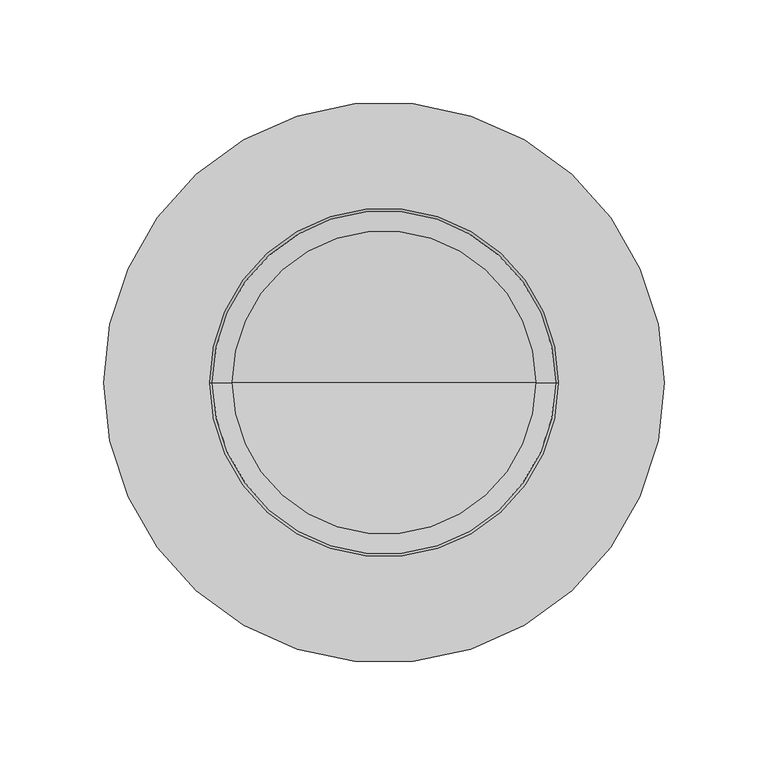
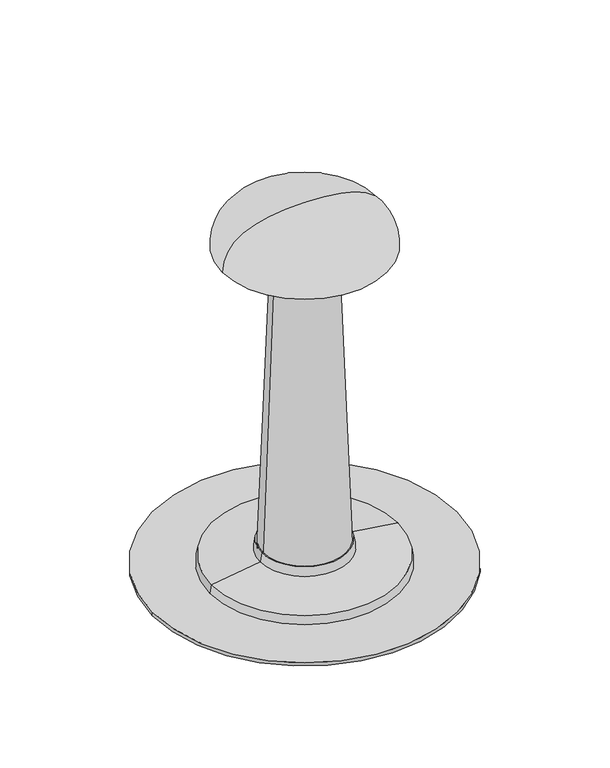
"""IFC4 building model written with IfcOpenShell, lengths in millimetres: proxy geometry, TN_Аэратор кровельный ТехноНИКОЛЬ ЭКО_Тип 1 : Аэратор кровельный ТехноНИКОЛЬ ЭКО 75х340мм."""

from ifc_helpers import new_model, si_unit, point, frame, origin, origin_with_axes, origin_2d, place, context, project, spatial, polyline, circle_curve, trimmed, segment, composite_curve, outline, extrude, source, transform, mapped, element, save
from ifc_brep_helpers import plane_surface, revolved_surface, spline_curve, advanced_brep


def specialty_equipment_94cada28(model_context):
    return source(origin(), model_context, "Body", "SolidModel", [
        advanced_brep(
        [(26.3779945, 0.0, 300.3783699), (-26.3779945, 0.0, 300.3783699), (0.0, 0.0, 300.3783699), (0.0, 0.0, 3.0), (-37.5, 0.0, 3.0), (37.5, 0.0, 3.0)],
        [
            (0, 1, circle_curve(frame((0.0, 0.0, 300.3783699), z_axis=(0.0, 0.0, 1.0), x_axis=(-1.0, 0.0, 0.0)), 26.3779945)),
            (1, 2),
            (2, 0),
            (1, 0, circle_curve(frame((0.0, 0.0, 300.3783699), z_axis=(0.0, 0.0, 1.0), x_axis=(-1.0, 0.0, 0.0)), 26.3779945)),
            (3, 4),
            (4, 5, circle_curve(frame((0.0, 0.0, 3.0), z_axis=(0.0, 0.0, -1.0), x_axis=(-1.0, 0.0, 0.0)), 37.5)),
            (5, 3),
            (5, 4, circle_curve(frame((0.0, 0.0, 3.0), z_axis=(0.0, 0.0, -1.0), x_axis=(-1.0, 0.0, 0.0)), 37.5)),
            (4, 1),
            (0, 5),
        ],
        [
            plane_surface(frame((0.0, 0.0, 300.3783699), z_axis=(0.0, 0.0, 1.0), x_axis=(-1.0, 0.0, 0.0))),
            plane_surface(frame((0.0, 0.0, 3.0), z_axis=(0.0, 0.0, -1.0), x_axis=(-1.0, 0.0, 0.0))),
            revolved_surface(polyline([(-26.3779945, 0.0, 300.3783699), (-37.5, 0.0, 3.0)]), (0.0, 0.0, 0.0), (0.0, 0.0, -1.0)),
        ],
        [
            (0, [[1, 2, 3]]),
            (0, [[4, -3, -2]]),
            (1, [[5, 6, 7]]),
            (1, [[-7, 8, -5]]),
            (2, [[-6, 9, -1, 10]]),
            (2, [[-8, -10, -4, -9]]),
        ],
    ),
        advanced_brep(
        [(0.0, 0.0, 300.3783699), (-73.0, 0.0, 300.3783699), (73.0, 0.0, 300.3783699), (0.0, 0.0, 340.3783699)],
        [
            (0, 1),
            (1, 2, circle_curve(frame((0.0, 0.0, 300.3783699), z_axis=(0.0, 0.0, -1.0), x_axis=(-1.0, 0.0, 0.0)), 73.0)),
            (2, 0),
            (2, 1, circle_curve(frame((0.0, 0.0, 300.3783699), z_axis=(0.0, 0.0, -1.0), x_axis=(-1.0, 0.0, 0.0)), 73.0)),
            (1, 3, spline_curve(3, [(-73.0, 0.0, 300.3783699), (-73.0, 0.0, 327.045036564), (-48.666666669, 0.0, 340.3783699), (0.0, 0.0, 340.3783699)], [4, 4], [0.0, 0.1853674540682417])),
            (3, 2, spline_curve(3, [(0.0, 0.0, 340.3783699), (48.666666669, 0.0, 340.3783699), (73.0, 0.0, 327.045036564), (73.0, 0.0, 300.3783699)], [4, 4], [0.0, 0.1853674540682417])),
        ],
        [
            plane_surface(frame((0.0, 0.0, 300.3783699), z_axis=(0.0, 0.0, -1.0), x_axis=(-1.0, 0.0, 0.0))),
            revolved_surface(spline_curve(3, [(0.0, 0.0, 340.3783699), (-48.666666669, 0.0, 340.3783699), (-73.0, 0.0, 327.045036564), (-73.0, 0.0, 300.3783699)], [4, 4], [0.0, 0.1853674540682417]), (0.0, 0.0, 340.3783699), (0.0, 0.0, -1.0)),
        ],
        [
            (0, [[1, 2, 3]]),
            (0, [[-3, 4, -1]]),
            (1, [[-2, 5, 6]]),
            (1, [[-4, -6, -5]]),
        ],
    ),
        advanced_brep(
        [(39.4106158, 0.0, 17.0), (-39.4106158, 0.0, 17.0), (-38.0, 0.0, 25.0), (38.0, 0.0, 25.0), (82.642123, 0.0, 10.7009033), (-82.642123, 0.0, 10.7009033), (84.0, 0.0, 3.0), (-84.0, 0.0, 3.0), (37.5, 0.0, 3.0), (-37.5, 0.0, 3.0), (-36.4162562, 0.0, 25.0), (36.4162562, 0.0, 25.0)],
        [
            (0, 1, circle_curve(frame((0.0, 0.0, 17.0), z_axis=(0.0, 0.0, 1.0), x_axis=(-1.0, 0.0, 0.0)), 39.4106158)),
            (1, 2),
            (2, 3, circle_curve(frame((0.0, 0.0, 25.0), z_axis=(0.0, 0.0, -1.0), x_axis=(-1.0, 0.0, 0.0)), 38.0)),
            (3, 0),
            (1, 0, circle_curve(frame((0.0, 0.0, 17.0), z_axis=(0.0, 0.0, 1.0), x_axis=(-1.0, 0.0, 0.0)), 39.4106158)),
            (3, 2, circle_curve(frame((0.0, 0.0, 25.0), z_axis=(0.0, 0.0, -1.0), x_axis=(-1.0, 0.0, 0.0)), 38.0)),
            (4, 5, circle_curve(frame((0.0, 0.0, 10.7009033), z_axis=(0.0, 0.0, 1.0), x_axis=(-1.0, 0.0, 0.0)), 82.642123)),
            (5, 1),
            (0, 4),
            (5, 4, circle_curve(frame((0.0, 0.0, 10.7009033), z_axis=(0.0, 0.0, 1.0), x_axis=(-1.0, 0.0, 0.0)), 82.642123)),
            (6, 7, circle_curve(frame((0.0, 0.0, 3.0), z_axis=(0.0, 0.0, 1.0), x_axis=(-1.0, 0.0, 0.0)), 84.0)),
            (7, 5),
            (4, 6),
            (7, 6, circle_curve(frame((0.0, 0.0, 3.0), z_axis=(0.0, 0.0, 1.0), x_axis=(-1.0, 0.0, 0.0)), 84.0)),
            (8, 9, circle_curve(frame((0.0, 0.0, 3.0), z_axis=(0.0, 0.0, 1.0), x_axis=(-1.0, 0.0, 0.0)), 37.5)),
            (9, 7),
            (6, 8),
            (9, 8, circle_curve(frame((0.0, 0.0, 3.0), z_axis=(0.0, 0.0, 1.0), x_axis=(-1.0, 0.0, 0.0)), 37.5)),
            (2, 10),
            (10, 11, circle_curve(frame((0.0, 0.0, 25.0), z_axis=(0.0, 0.0, -1.0), x_axis=(-1.0, 0.0, 0.0)), 36.4162562)),
            (11, 3),
            (11, 10, circle_curve(frame((0.0, 0.0, 25.0), z_axis=(0.0, 0.0, -1.0), x_axis=(-1.0, 0.0, 0.0)), 36.4162562)),
            (10, 9),
            (8, 11),
        ],
        [
            revolved_surface(polyline([(-38.0, 0.0, 25.0), (-39.4106158, 0.0, 17.0)]), (0.0, 0.0, 0.0), (0.0, 0.0, -1.0)),
            revolved_surface(polyline([(-39.4106158, 0.0, 17.0), (-82.642123, 0.0, 10.7009033)]), (0.0, 0.0, 0.0), (0.0, 0.0, -1.0)),
            revolved_surface(polyline([(-82.642123, 0.0, 10.7009033), (-84.0, 0.0, 3.0)]), (0.0, 0.0, 0.0), (0.0, 0.0, -1.0)),
            plane_surface(frame((0.0, 0.0, 3.0), z_axis=(0.0, 0.0, -1.0), x_axis=(-1.0, 0.0, 0.0))),
            plane_surface(frame((0.0, 0.0, 25.0), z_axis=(0.0, 0.0, 1.0), x_axis=(-1.0, 0.0, 0.0))),
            revolved_surface(polyline([(-37.5, 0.0, 3.0), (-36.4162562, 0.0, 25.0)]), (0.0, 0.0, 0.0), (0.0, 0.0, -1.0)),
        ],
        [
            (0, [[1, 2, 3, 4]]),
            (0, [[5, -4, 6, -2]]),
            (1, [[7, 8, -1, 9]]),
            (1, [[10, -9, -5, -8]]),
            (2, [[11, 12, -7, 13]]),
            (2, [[14, -13, -10, -12]]),
            (3, [[15, 16, -11, 17]]),
            (3, [[18, -17, -14, -16]]),
            (4, [[-3, 19, 20, 21]]),
            (4, [[-6, -21, 22, -19]]),
            (5, [[-20, 23, -15, 24]]),
            (5, [[-22, -24, -18, -23]]),
        ],
    ),
        extrude(outline(composite_curve([segment(trimmed(circle_curve(origin_2d(), 135.0), [point((-135.0, 0.0))], [point((135.0, 0.0))], False, "CARTESIAN"), True, "CONTINUOUS"), segment(trimmed(circle_curve(origin_2d(), 135.0), [point((135.0, 0.0))], [point((-135.0, 0.0))], False, "CARTESIAN"), True, "CONTINUOUS")], self_intersect=False)), origin_with_axes(), (0.0, 0.0, 1.0), 3.0),
    ])


if __name__ == "__main__":
    model = new_model("IFC4")
    model_context = context("Model", 3, world=origin())
    ifc_project = project(units=[si_unit("LENGTHUNIT", "METRE", prefix="MILLI")], contexts=[model_context])
    site = spatial("IfcSite", under=ifc_project)
    building = spatial("IfcBuilding", under=site)
    placement = place(None, origin())
    specialty_equipment_shape = specialty_equipment_94cada28(model_context)
    element("IfcBuildingElementProxy", 1, Name="TN_Аэратор кровельный ТехноНИКОЛЬ ЭКО_Тип 1 : Аэратор кровельный ТехноНИКОЛЬ ЭКО 75х340мм", ObjectType="TN_Аэратор кровельный ТехноНИКОЛЬ ЭКО_Тип 1 : Аэратор кровельный ТехноНИКОЛЬ ЭКО 75х340мм", at=placement, inside=building, context=model_context, shape_type="MappedRepresentation", body=[
        mapped(specialty_equipment_shape, transform((0.0, 0.0, 0.0), x_axis=(1.0, 0.0, 0.0), y_axis=(0.0, 1.0, 0.0), z_axis=(0.0, 0.0, 1.0))),
    ])
    save(model, "model.ifc")

# Revit data of these elements
# Type "TN_Аэратор кровельный ТехноНИКОЛЬ ЭКО_Тип 1 : Аэратор кровельный ТехноНИКОЛЬ ЭКО 75х340мм"
#   Description = "Аэратор кровельный ТехноНИКОЛЬ ЭКО 75х340 мм может быть использован только при\r\nремонтах кровли. Аэродинамическая форма и уменьшенное проходное сечение позволяют ему работать только после\r\nдостаточно сильного прогрева кровли. Устанавливается 1 на 100 м2 вне зависимости от способа монтажа кровли и\r\nпредотвращает только образование вздутий под кровлей. Его конструкция не подразумевает доутепления\r\nкерамзитовым гравием.\r\nКровельные аэраторы запрещено устанавливать в совмещенных кровлях над холодильниками и ледовыми аренами."
#   Manufacturer = "ТехноНИКОЛЬ"
#   URL = "https://shop.tn.ru/ajerator-krovel-nyj-tehnonikol-jeko-75h340-mm"
#   ADSK_Примечание = ""
#   ADSK_Обозначение = "ТехноНИКОЛЬ"
#   ADSK_Наименование = "Аэратор кровельный ТехноНИКОЛЬ ЭКО 75х340мм"
#   ADSK_Марка = ""
#   ADSK_Код изделия = "5489"
#   ADSK_Завод-изготовитель = "ТехноНИКОЛЬ"
#   ADSK_Единица измерения = "шт."
#   ADSK_Группирование = "Комплектующие и воронки"
#   ADSK_URL страницы изделия = "https://shop.tn.ru/ajerator-krovel-nyj-tehnonikol-jeko-75h340-mm#documents"
#   ADSK_URL документации изделия = "https://nav.tn.ru/upload/iblock/68a/Tekhlist-7.18_Aerator-krovelnyy-TekhnoNIKOL_rus.pdf"
#   ADSK_Масса = 0.3
#   ADSK_Количество = 1
#   Материал = TN_ПВХ_Черный
#   Default Elevation = 0
# Element 1 (IfcBuildingElementProxy, "TN_Аэратор кровельный ТехноНИКОЛЬ ЭКО_Тип 1 : Аэратор кровельный ТехноНИКОЛЬ ЭКО 75х340мм")
#   Materials on its faces: "TN_ПВХ_Черный"
# Materials
#   "TN_ПВХ_Черный": class "Типовые", colour RGB 48 48 48, transparency 0, Cost = 0
